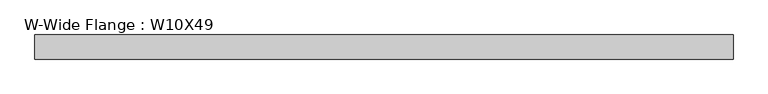
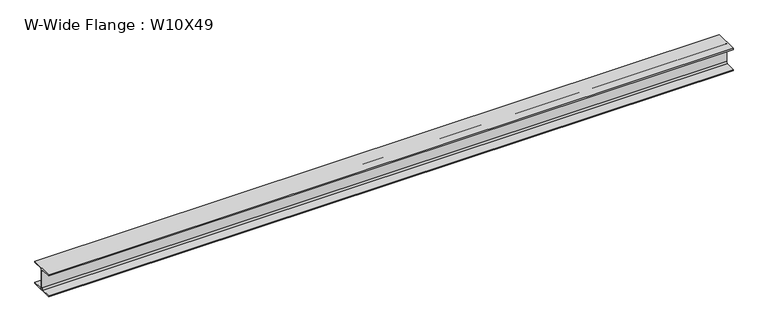
"""IFC4 building model written with IfcOpenShell, lengths in millimetres: beam geometry, W-Wide Flange : W10X49."""

from ifc_helpers import new_model, si_unit, point, frame, frame_2d, origin, place, context, project, spatial, polyline, circle_curve, trimmed, segment, composite_curve, outline, extrude, source, transform, mapped, element, save


def w_wide_flange_w10x49_96518129(model_context):
    return source(origin(), model_context, "Body", "SweptSolid", [
        extrude(outline(composite_curve([segment(polyline([(127.0, -112.776), (127.0, -127.0), (-127.0, -127.0), (-127.0, -112.776), (-21.844, -112.776)]), True, "CONTINUOUS"), segment(trimmed(circle_curve(frame_2d((-21.844, -95.25)), 17.526), [point((-21.844, -112.776))], [point((-4.318, -95.25))], True, "CARTESIAN"), True, "CONTINUOUS"), segment(polyline([(-4.318, -95.25), (-4.318, 95.25)]), True, "CONTINUOUS"), segment(trimmed(circle_curve(frame_2d((-21.844, 95.25)), 17.526), [point((-4.318, 95.25))], [point((-21.844, 112.776))], True, "CARTESIAN"), True, "CONTINUOUS"), segment(polyline([(-21.844, 112.776), (-127.0, 112.776), (-127.0, 127.0), (127.0, 127.0), (127.0, 112.776), (21.844, 112.776)]), True, "CONTINUOUS"), segment(trimmed(circle_curve(frame_2d((21.844, 95.25)), 17.526), [point((21.844, 112.776))], [point((4.318, 95.25))], True, "CARTESIAN"), True, "CONTINUOUS"), segment(polyline([(4.318, 95.25), (4.318, -95.25)]), True, "CONTINUOUS"), segment(trimmed(circle_curve(frame_2d((21.844, -95.25)), 17.526), [point((4.318, -95.25))], [point((21.844, -112.776))], True, "CARTESIAN"), True, "CONTINUOUS"), segment(polyline([(21.844, -112.776), (127.0, -112.776)]), True, "CONTINUOUS")], self_intersect=False)), frame((-3648.0253906, 0.0, 0.0), z_axis=(1.0, 0.0, 0.0), x_axis=(0.0, 1.0, 0.0)), (0.0, 0.0, 1.0), 7358.7570312),
    ])


if __name__ == "__main__":
    model = new_model("IFC4")
    model_context = context("Model", 3, world=origin())
    ifc_project = project(units=[si_unit("LENGTHUNIT", "METRE", prefix="MILLI")], contexts=[model_context])
    site = spatial("IfcSite", under=ifc_project)
    building = spatial("IfcBuilding", under=site)
    placement = place(None, origin())
    w_wide_flange_w10x49_shape = w_wide_flange_w10x49_96518129(model_context)
    element("IfcBeam", 1, ObjectType="W-Wide Flange : W10X49", at=placement, inside=building, context=model_context, shape_type="MappedRepresentation", body=[
        mapped(w_wide_flange_w10x49_shape, transform((0.0, 0.0, 0.0), x_axis=(1.0, 0.0, 0.0), y_axis=(0.0, 1.0, 0.0), z_axis=(0.0, 0.0, 1.0))),
    ])
    save(model, "model.ifc")

# Revit data of these elements
# Type "W-Wide Flange : W10X49"
#   Assembly Code = "B10"
#   W = 49
#   Length [instance default] = 1524 mm
#   bf = 254 mm
#   d = 254 mm
#   k = 31.75 mm
#   k2 = 17.526 mm
#   tf = 14.224 mm
#   tw = 8.636 mm
#   A = 0.0092903 m²
#   Structural Material [instance default] = Steel ASTM A992
# Element 1 (IfcBeam, "W-Wide Flange : W10X49")
#   Structural Material = Aluminum, Anodized Red
#   Materials on its faces: "Aluminum, Anodized Red"
# Materials
#   "Steel ASTM A992": class "Metal", colour RGB 128 0 0, transparency 0, Description = "Structural steel 50ksi", Cost = 0
#   "Aluminum, Anodized Red": class "Metal", colour RGB 120 120 120, transparency 0, Description = "Anodized aluminum, red", Cost = 0
